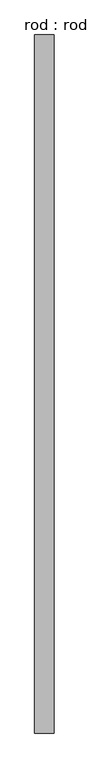
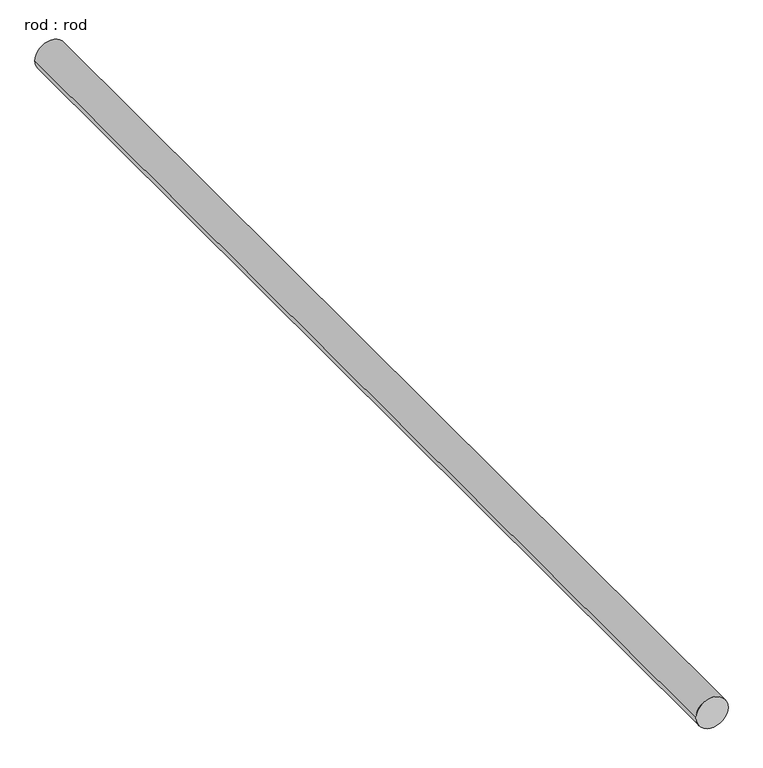
"""IFC4 building model written with IfcOpenShell, lengths in millimetres: proxy geometry, rod : rod."""

from ifc_helpers import new_model, si_unit, point, frame, frame_2d, origin, place, context, project, spatial, circle_curve, trimmed, segment, composite_curve, outline, extrude, source, transform, mapped, element, save


def rod_rod_39824f73(model_context):
    return source(origin(), model_context, "Body", "SweptSolid", [
        extrude(outline(composite_curve([segment(trimmed(circle_curve(frame_2d((0.0108462, 0.0)), 200.0), [point((0.0108462, 200.0))], [point((0.0108462, -200.0))], False, "CARTESIAN"), True, "CONTINUOUS"), segment(trimmed(circle_curve(frame_2d((0.0108462, 0.0)), 200.0), [point((0.0108462, -200.0))], [point((0.0108462, 200.0))], False, "CARTESIAN"), True, "CONTINUOUS")], self_intersect=False)), frame((0.0, -3046.1602736, 0.0), z_axis=(0.0, 1.0, 0.0), x_axis=(0.0, 0.0, 1.0)), (0.0, 0.0, 1.0), 14277.7777778),
    ])


if __name__ == "__main__":
    model = new_model("IFC4")
    model_context = context("Model", 3, world=origin())
    ifc_project = project(units=[si_unit("LENGTHUNIT", "METRE", prefix="MILLI")], contexts=[model_context])
    site = spatial("IfcSite", under=ifc_project)
    building = spatial("IfcBuilding", under=site)
    placement = place(None, origin())
    rod_rod_shape = rod_rod_39824f73(model_context)
    element("IfcBuildingElementProxy", 1, Name="rod : rod", ObjectType="rod : rod", at=placement, inside=building, context=model_context, shape_type="MappedRepresentation", body=[
        mapped(rod_rod_shape, transform((0.0, 0.0, 0.0), x_axis=(1.0, 0.0, 0.0), y_axis=(0.0, 1.0, 0.0), z_axis=(0.0, 0.0, 1.0))),
    ])
    save(model, "model.ifc")

# Revit data of these elements
# Type "rod : rod"
#   Default Elevation = 0
